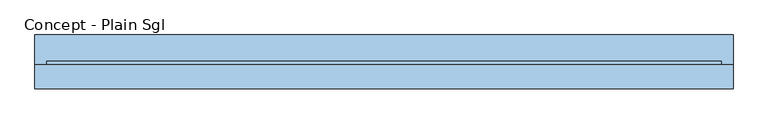
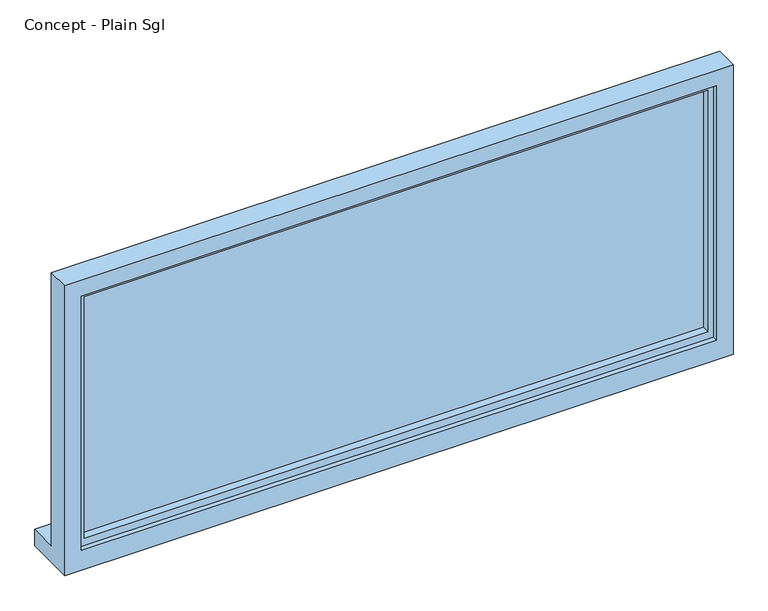
"""IFC4 building model written with IfcOpenShell, lengths in millimetres: window geometry, Concept - Plain Sgl : Visiuon Panel no Opening Sashes."""

from ifc_helpers import new_model, si_unit, frame, origin, place, context, project, spatial, polyline, outline, extrude, faceted_brep, source, transform, mapped, element, save


def concept_plain_sgl_1110da93(model_context):
    return source(origin(), model_context, "Body", "SolidModel", [
        faceted_brep([(-1200.0, -27.0434322, 1010.0), (1200.0, -27.0434322, 1010.0), (1200.0, -27.0434322, 2110.0), (-1200.0, -27.0434322, 2110.0), (-1140.0, -27.0434322, 2050.0), (1140.0, -27.0434322, 2050.0), (1140.0, -27.0434322, 1085.0), (-1140.0, -27.0434322, 1085.0), (-1200.0, 55.9565678, 2110.0), (-1200.0, 55.9565678, 1073.0), (-1200.0, 158.4565678, 1073.0), (-1200.0, 158.4565678, 1010.0), (1200.0, 55.9565678, 2110.0), (1200.0, 55.9565678, 1073.0), (1160.0, 55.9565678, 1073.0), (1160.0, 55.9565678, 2070.0), (-1160.0, 55.9565678, 2070.0), (-1160.0, 55.9565678, 1073.0), (-1160.0, -9.0434322, 2070.0), (-1160.0, -9.0434322, 1073.0), (1160.0, -9.0434322, 2070.0), (1160.0, -9.0434322, 1073.0), (-1140.0, -9.0434322, 2050.0), (-1140.0, -9.0434322, 1085.0), (1140.0, -9.0434322, 1085.0), (1140.0, -9.0434322, 2050.0), (1200.0, 158.4565678, 1010.0), (1200.0, 158.4565678, 1073.0)], [[[0, 1, 2, 3], [4, 5, 6, 7]], [[0, 3, 8, 9, 10, 11]], [[9, 8, 12, 13, 14, 15, 16, 17]], [[17, 16, 18, 19]], [[18, 20, 21, 19], [22, 23, 24, 25]], [[22, 4, 7, 23]], [[3, 2, 12, 8]], [[16, 15, 20, 18]], [[5, 4, 22, 25]], [[13, 12, 2, 1, 26, 27]], [[15, 14, 21, 20]], [[5, 25, 24, 6]], [[26, 1, 0, 11]], [[27, 26, 11, 10]], [[27, 10, 9, 17, 19, 21, 14, 13]], [[7, 6, 24, 23]]]),
        extrude(outline(polyline([(1130.0, 19.9565678), (-1130.0, 19.9565678), (-1130.0, 43.9565678), (1130.0, 43.9565678), (1130.0, 19.9565678)])), frame((0.0, 0.0, 1103.0), z_axis=(0.0, 0.0, 1.0), x_axis=(1.0, 0.0, 0.0)), (0.0, 0.0, 1.0), 937.0),
        faceted_brep([(-1160.0, -9.0434322, 2070.0), (-1160.0, 67.5035732, 2070.0), (-1160.0, 67.5035732, 1073.0), (-1160.0, -9.0434322, 1073.0), (-1120.0, 19.9565678, 2030.0), (-1120.0, -9.0434322, 2030.0), (-1120.0, -9.0434322, 1113.0), (-1120.0, 19.9565678, 1113.0), (-1130.0, 43.9565678, 2040.0), (-1130.0, 19.9565678, 2040.0), (-1130.0, 19.9565678, 1103.0), (-1130.0, 43.9565678, 1103.0), (-1120.0, 67.5035732, 2030.0), (-1120.0, 43.9565678, 2030.0), (-1120.0, 43.9565678, 1113.0), (-1120.0, 67.5035732, 1113.0), (1160.0, 67.5035732, 1073.0), (1160.0, -9.0434322, 1073.0), (1120.0, -9.0434322, 1113.0), (1120.0, 19.9565678, 1113.0), (1130.0, 19.9565678, 1103.0), (1130.0, 43.9565678, 1103.0), (1120.0, 43.9565678, 1113.0), (1120.0, 67.5035732, 1113.0), (1160.0, 67.5035732, 2070.0), (1160.0, -9.0434322, 2070.0), (1120.0, -9.0434322, 2030.0), (1120.0, 19.9565678, 2030.0), (1130.0, 19.9565678, 2040.0), (1130.0, 43.9565678, 2040.0), (1120.0, 43.9565678, 2030.0), (1120.0, 67.5035732, 2030.0)], [[[0, 1, 2, 3]], [[4, 5, 6, 7]], [[8, 9, 10, 11]], [[12, 13, 14, 15]], [[3, 2, 16, 17]], [[7, 6, 18, 19]], [[11, 10, 20, 21]], [[15, 14, 22, 23]], [[17, 16, 24, 25]], [[19, 18, 26, 27]], [[21, 20, 28, 29]], [[23, 22, 30, 31]], [[1, 24, 16, 2], [15, 23, 31, 12]], [[25, 24, 1, 0]], [[3, 17, 25, 0], [5, 26, 18, 6]], [[27, 26, 5, 4]], [[9, 28, 20, 10], [7, 19, 27, 4]], [[29, 28, 9, 8]], [[11, 21, 29, 8], [13, 30, 22, 14]], [[31, 30, 13, 12]]]),
    ])


if __name__ == "__main__":
    model = new_model("IFC4")
    model_context = context("Model", 3, world=origin())
    ifc_project = project(units=[si_unit("LENGTHUNIT", "METRE", prefix="MILLI")], contexts=[model_context])
    site = spatial("IfcSite", under=ifc_project)
    building = spatial("IfcBuilding", under=site)
    placement = place(None, origin())
    concept_plain_sgl_shape = concept_plain_sgl_1110da93(model_context)
    element("IfcWindow", 1, ObjectType="Concept - Plain Sgl : Visiuon Panel no Opening Sashes", at=placement, inside=building, context=model_context, shape_type="MappedRepresentation", body=[
        mapped(concept_plain_sgl_shape, transform((0.0, 0.0, 0.0), x_axis=(1.0, 0.0, 0.0), y_axis=(0.0, 1.0, 0.0), z_axis=(0.0, 0.0, 1.0))),
    ])
    save(model, "model.ifc")

# Revit data of these elements
# Project information
#   Document_Suitability_Code = "A1"
#   Document_Suitability_Description = "Coordination"
#   Project Status = "Project Status"
#   Client Name = "Revit Project"
#   Project Address = "Limerick Institute of Technology"
#   Project Name = "Commercial Units"
#   Project Number = "RARC02"
# Type "Concept - Plain Sgl : Visiuon Panel no Opening Sashes"
#   Type Mark = "44"
#   Operation = "SinglePanel"
#   Description = "Half Hour Vision Panel"
#   Manufacturer = "Revit"
#   Keynote = "L10"
#   Visual Light Transmittance = 0.9
#   Solar Heat Gain Coefficient = 0.86
#   Rough Width = 2400 mm
#   Rough Height = 1100 mm
#   Height = 1100 mm
#   Width = 2400 mm
#   Heat Transfer Coefficient (U) = 5.5617 W/(m²·K)
#   FrameOffset - External = 0 mm
#   Default Head Height = 2110 mm
#   Define Thermal Properties by = 1
#   Material Trim = Window Frame
#   Material Glass = Glass
#   Material Frame = Window Frame
#   Construction Type Id = ""
#   Wall Closure = (empty or 0)
#   Analytic Construction = (empty or 0)
# Element 1 (IfcWindow, "Concept - Plain Sgl : Visiuon Panel no Opening Sashes")
#   Materials on its faces: "Window Frame", "Glass"
# Materials
#   "Window Frame": class "Miscellaneous", colour RGB 249 249 249, transparency 0, Keynote = "L10"
#   "Glass": class "Glass", colour RGB 0 128 192, transparency 0.9, Description = "Soda Lime Glass", Cost = 0
